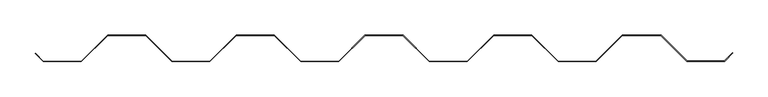
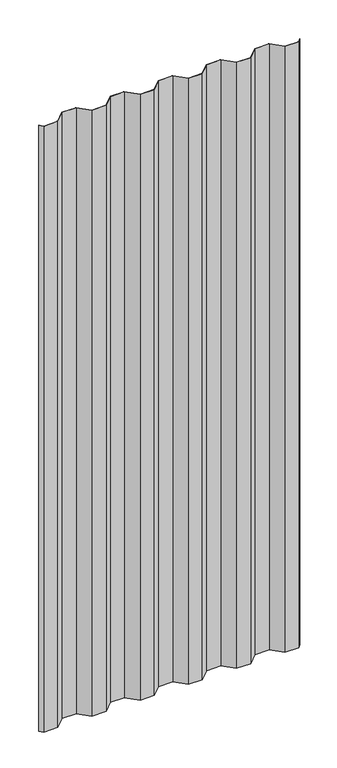
"""IFC4 building model written with IfcOpenShell, lengths in millimetres: proxy geometry, MBCI 7.2-V Panel12 : MBCI 7.2-V Panel-1."""

from ifc_helpers import new_model, si_unit, frame, origin, place, context, project, spatial, polyline, outline, extrude, source, transform, mapped, element, save


def generic_models_de5cb4ec(model_context):
    return source(origin(), model_context, "Body", "SweptSolid", [
        extrude(outline(polyline([(589155.5303729, -531639.2163841), (589101.4186638, -531639.2163841), (589090.0180296, -531627.81575), (589090.8180038, -531627.7738251), (589101.6652503, -531638.6210716), (589155.2837864, -531638.6210716), (589192.7741864, -531601.1306716), (589247.0548503, -531601.1306716), (589284.5452503, -531638.6210716), (589338.1637864, -531638.6210716), (589375.6541864, -531601.1306716), (589429.9348503, -531601.1306716), (589467.4252503, -531638.6210716), (589521.0437864, -531638.6210716), (589558.5341864, -531601.1306716), (589612.8148503, -531601.1306716), (589650.3052503, -531638.6210716), (589703.9237864, -531638.6210716), (589741.4141864, -531601.1306716), (589795.6948503, -531601.1306716), (589833.1852503, -531638.6210716), (589886.8037864, -531638.6210716), (589924.2941864, -531601.1306716), (589979.4384503, -531601.1306716), (590016.3192503, -531638.0114716), (590069.4073773, -531638.0114716), (590080.5378112, -531626.8810377), (590081.3246865, -531626.9360614), (590069.6539638, -531638.6067841), (590016.0726638, -531638.6067841), (589979.1918638, -531601.7259841), (589924.5407729, -531601.7259841), (589887.0503729, -531639.2163841), (589832.9386638, -531639.2163841), (589795.4482638, -531601.7259841), (589741.6607729, -531601.7259841), (589704.1703729, -531639.2163841), (589650.0586638, -531639.2163841), (589612.5682638, -531601.7259841), (589558.7807729, -531601.7259841), (589521.2903729, -531639.2163841), (589467.1786638, -531639.2163841), (589429.6882638, -531601.7259841), (589375.9007729, -531601.7259841), (589338.4103729, -531639.2163841), (589284.2986638, -531639.2163841), (589246.8082638, -531601.7259841), (589193.0207729, -531601.7259841), (589155.5303729, -531639.2163841)])), frame((0.0, 0.0, 6.35), z_axis=(0.0, 0.0, 1.0), x_axis=(1.0, 0.0, 0.0)), (0.0, 0.0, 1.0), 2432.05),
    ])


if __name__ == "__main__":
    model = new_model("IFC4")
    model_context = context("Model", 3, world=origin())
    ifc_project = project(units=[si_unit("LENGTHUNIT", "METRE", prefix="MILLI")], contexts=[model_context])
    site = spatial("IfcSite", under=ifc_project)
    building = spatial("IfcBuilding", under=site)
    placement = place(None, origin())
    generic_models_shape = generic_models_de5cb4ec(model_context)
    element("IfcBuildingElementProxy", 1, Name="MBCI 7.2-V Panel12 : MBCI 7.2-V Panel-1", ObjectType="MBCI 7.2-V Panel12 : MBCI 7.2-V Panel-1", at=placement, inside=building, context=model_context, shape_type="MappedRepresentation", body=[
        mapped(generic_models_shape, transform((0.0, 0.0, 0.0), x_axis=(1.0, 0.0, 0.0), y_axis=(0.0, 1.0, 0.0), z_axis=(0.0, 0.0, 1.0))),
    ])
    save(model, "model.ifc")

# Revit data of these elements
# Element 1 (IfcBuildingElementProxy, "MBCI 7.2-V Panel12 : MBCI 7.2-V Panel-1")
#   Materials on its faces: "MTL PANEL"
# Materials
#   "MTL PANEL": class "Generic", colour RGB 239 242 240, transparency 0, Cost = 0
